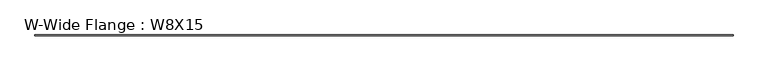
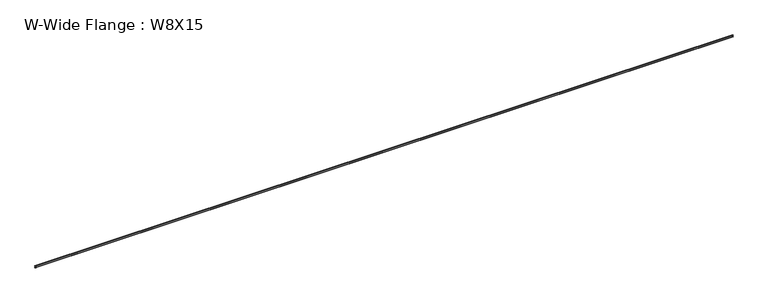
"""IFC4 building model written with IfcOpenShell, lengths in millimetres: beam geometry, W-Wide Flange : W8X15."""

from ifc_helpers import new_model, si_unit, point, frame, frame_2d, origin, place, context, project, spatial, polyline, circle_curve, trimmed, segment, composite_curve, outline, extrude, source, transform, mapped, element, save


def w_wide_flange_w8x15_5bedcf3e(model_context):
    return source(origin(), model_context, "Body", "SweptSolid", [
        extrude(outline(composite_curve([segment(polyline([(50.927, -94.996), (50.927, -102.997), (-50.927, -102.997), (-50.927, -94.996), (-15.748, -94.996)]), True, "CONTINUOUS"), segment(trimmed(circle_curve(frame_2d((-15.748, -82.3595)), 12.6365), [point((-15.748, -94.996))], [point((-3.1115, -82.3595))], True, "CARTESIAN"), True, "CONTINUOUS"), segment(polyline([(-3.1115, -82.3595), (-3.1115, 82.3595)]), True, "CONTINUOUS"), segment(trimmed(circle_curve(frame_2d((-15.748, 82.3595)), 12.6365), [point((-3.1115, 82.3595))], [point((-15.748, 94.996))], True, "CARTESIAN"), True, "CONTINUOUS"), segment(polyline([(-15.748, 94.996), (-50.927, 94.996), (-50.927, 102.997), (50.927, 102.997), (50.927, 94.996), (15.748, 94.996)]), True, "CONTINUOUS"), segment(trimmed(circle_curve(frame_2d((15.748, 82.3595)), 12.6365), [point((15.748, 94.996))], [point((3.1115, 82.3595))], True, "CARTESIAN"), True, "CONTINUOUS"), segment(polyline([(3.1115, 82.3595), (3.1115, -82.3595)]), True, "CONTINUOUS"), segment(trimmed(circle_curve(frame_2d((15.748, -82.3595)), 12.6365), [point((3.1115, -82.3595))], [point((15.748, -94.996))], True, "CARTESIAN"), True, "CONTINUOUS"), segment(polyline([(15.748, -94.996), (50.927, -94.996)]), True, "CONTINUOUS")], self_intersect=False)), frame((-44059.871875, 0.0, 0.0), z_axis=(1.0, 0.0, 0.0), x_axis=(0.0, 1.0, 0.0)), (0.0, 0.0, 1.0), 88017.35),
    ])


if __name__ == "__main__":
    model = new_model("IFC4")
    model_context = context("Model", 3, world=origin())
    ifc_project = project(units=[si_unit("LENGTHUNIT", "METRE", prefix="MILLI")], contexts=[model_context])
    site = spatial("IfcSite", under=ifc_project)
    building = spatial("IfcBuilding", under=site)
    placement = place(None, origin())
    w_wide_flange_w8x15_shape = w_wide_flange_w8x15_5bedcf3e(model_context)
    element("IfcBeam", 1, ObjectType="W-Wide Flange : W8X15", at=placement, inside=building, context=model_context, shape_type="MappedRepresentation", body=[
        mapped(w_wide_flange_w8x15_shape, transform((0.0, 0.0, 0.0), x_axis=(1.0, 0.0, 0.0), y_axis=(0.0, 1.0, 0.0), z_axis=(0.0, 0.0, 1.0))),
    ])
    save(model, "model.ifc")

# Revit data of these elements
# Type "W-Wide Flange : W8X15"
#   Assembly Code = "B10"
#   W = 15
#   Length [instance default] = 5' - 0"
#   bf = 0' - 4.01"
#   d = 0' - 8.11"
#   k = 0' - 0 13/16"
#   k2 = 0' - 0.4975"
#   tf = 0' - 0.315"
#   tw = 0' - 0.245"
#   A = 0.0308333 SF
#   Structural Material [instance default] = Steel ASTM A992
# Element 1 (IfcBeam, "W-Wide Flange : W8X15")
#   Materials on its faces: "Steel ASTM A992"
# Materials
#   "Steel ASTM A992": class "Metal", colour RGB 199 199 199, transparency 0, Description = "Structural steel 50ksi", Cost = 0
